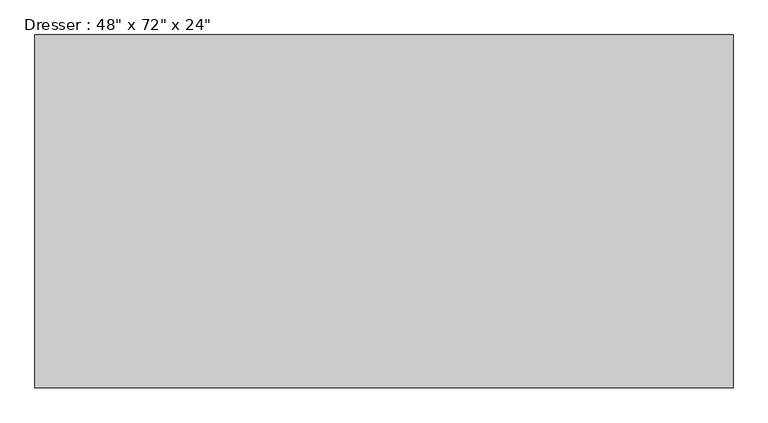
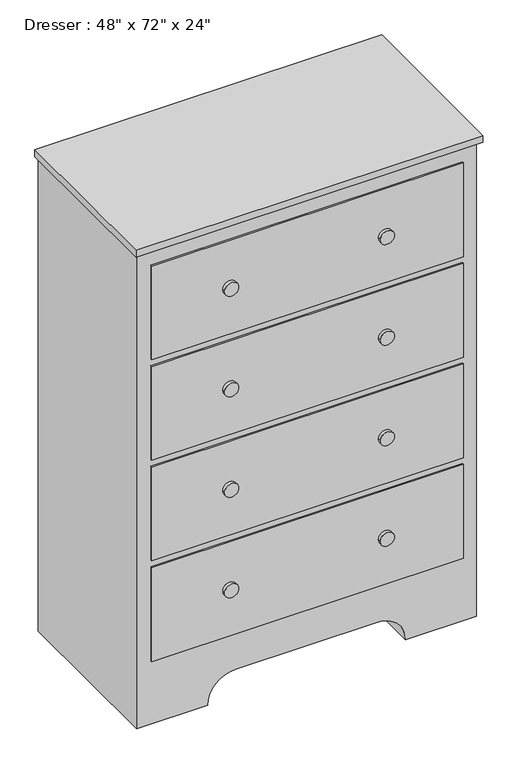
"""IFC4 building model written with IfcOpenShell, lengths in millimetres: furniture geometry."""

from ifc_helpers import new_model, si_unit, point, frame, frame_2d, origin, place, context, project, spatial, polyline, circle_curve, trimmed, segment, composite_curve, outline, extrude, source, transform, mapped, element, save


def furniture_c196debe(model_context):
    return source(origin(), model_context, "Body", "SweptSolid", [
        extrude(outline(composite_curve([segment(polyline([(0.0, 340.4067402), (1803.4, 340.4067402), (1803.4, -878.7932598), (0.0, -878.7932598), (0.0, -624.7932598)]), True, "CONTINUOUS"), segment(trimmed(circle_curve(frame_2d((0.0, -523.1932598)), 101.6), [point((0.0, -624.7932598))], [point((101.6, -523.1932598))], True, "CARTESIAN"), True, "CONTINUOUS"), segment(polyline([(101.6, -523.1932598), (101.6, -15.1932598)]), True, "CONTINUOUS"), segment(trimmed(circle_curve(frame_2d((0.0, -15.1932598)), 101.6), [point((101.6, -15.1932598))], [point((0.0, 86.4067402))], True, "CARTESIAN"), True, "CONTINUOUS"), segment(polyline([(0.0, 86.4067402), (0.0, 340.4067402)]), True, "CONTINUOUS")], self_intersect=False)), frame((0.0, -667.9629541, 0.0), z_axis=(0.0, 1.0, 0.0), x_axis=(0.0, 0.0, 1.0)), (0.0, 0.0, 1.0), 609.6),
        extrude(outline(polyline([(353.1067402, -58.3629541), (353.1067402, -687.0129541), (-891.4932598, -687.0129541), (-891.4932598, -58.3629541), (353.1067402, -58.3629541)])), frame((0.0, 0.0, 1803.4), z_axis=(0.0, 0.0, 1.0), x_axis=(1.0, 0.0, 0.0)), (0.0, 0.0, 1.0), 25.4),
        extrude(outline(polyline([(289.6067402, -674.3129541), (-827.9932598, -674.3129541), (-827.9932598, -667.9629541), (289.6067402, -667.9629541), (289.6067402, -674.3129541)])), frame((0.0, 0.0, 1384.3), z_axis=(0.0, 0.0, 1.0), x_axis=(1.0, 0.0, 0.0)), (0.0, 0.0, 1.0), 355.6),
        extrude(outline(polyline([(289.6067402, -674.3129541), (-827.9932598, -674.3129541), (-827.9932598, -667.9629541), (289.6067402, -667.9629541), (289.6067402, -674.3129541)])), frame((0.0, 0.0, 1003.3), z_axis=(0.0, 0.0, 1.0), x_axis=(1.0, 0.0, 0.0)), (0.0, 0.0, 1.0), 355.6),
        extrude(outline(polyline([(289.6067402, -674.3129541), (-827.9932598, -674.3129541), (-827.9932598, -667.9629541), (289.6067402, -667.9629541), (289.6067402, -674.3129541)])), frame((0.0, 0.0, 622.3), z_axis=(0.0, 0.0, 1.0), x_axis=(1.0, 0.0, 0.0)), (0.0, 0.0, 1.0), 355.6),
        extrude(outline(polyline([(289.6067402, -674.3129541), (-827.9932598, -674.3129541), (-827.9932598, -667.9629541), (289.6067402, -667.9629541), (289.6067402, -674.3129541)])), frame((0.0, 0.0, 241.3), z_axis=(0.0, 0.0, 1.0), x_axis=(1.0, 0.0, 0.0)), (0.0, 0.0, 1.0), 355.6),
        extrude(outline(composite_curve([segment(trimmed(circle_curve(frame_2d((1562.1, 10.2067402)), 25.4), [point((1562.1, -15.1932598))], [point((1562.1, 35.6067402))], False, "CARTESIAN"), True, "CONTINUOUS"), segment(trimmed(circle_curve(frame_2d((1562.1, 10.2067402)), 25.4), [point((1562.1, 35.6067402))], [point((1562.1, -15.1932598))], False, "CARTESIAN"), True, "CONTINUOUS")], self_intersect=False)), frame((0.0, -687.0129541, 0.0), z_axis=(0.0, 1.0, 0.0), x_axis=(0.0, 0.0, 1.0)), (0.0, 0.0, 1.0), 12.7),
        extrude(outline(composite_curve([segment(trimmed(circle_curve(frame_2d((1181.1, 10.2067402)), 25.4), [point((1181.1, -15.1932598))], [point((1181.1, 35.6067402))], False, "CARTESIAN"), True, "CONTINUOUS"), segment(trimmed(circle_curve(frame_2d((1181.1, 10.2067402)), 25.4), [point((1181.1, 35.6067402))], [point((1181.1, -15.1932598))], False, "CARTESIAN"), True, "CONTINUOUS")], self_intersect=False)), frame((0.0, -687.0129541, 0.0), z_axis=(0.0, 1.0, 0.0), x_axis=(0.0, 0.0, 1.0)), (0.0, 0.0, 1.0), 12.7),
        extrude(outline(composite_curve([segment(trimmed(circle_curve(frame_2d((800.1, 10.2067402)), 25.4), [point((800.1, -15.1932598))], [point((800.1, 35.6067402))], False, "CARTESIAN"), True, "CONTINUOUS"), segment(trimmed(circle_curve(frame_2d((800.1, 10.2067402)), 25.4), [point((800.1, 35.6067402))], [point((800.1, -15.1932598))], False, "CARTESIAN"), True, "CONTINUOUS")], self_intersect=False)), frame((0.0, -687.0129541, 0.0), z_axis=(0.0, 1.0, 0.0), x_axis=(0.0, 0.0, 1.0)), (0.0, 0.0, 1.0), 12.7),
        extrude(outline(composite_curve([segment(trimmed(circle_curve(frame_2d((419.1, 10.2067402)), 25.4), [point((419.1, -15.1932598))], [point((419.1, 35.6067402))], False, "CARTESIAN"), True, "CONTINUOUS"), segment(trimmed(circle_curve(frame_2d((419.1, 10.2067402)), 25.4), [point((419.1, 35.6067402))], [point((419.1, -15.1932598))], False, "CARTESIAN"), True, "CONTINUOUS")], self_intersect=False)), frame((0.0, -687.0129541, 0.0), z_axis=(0.0, 1.0, 0.0), x_axis=(0.0, 0.0, 1.0)), (0.0, 0.0, 1.0), 12.7),
        extrude(outline(composite_curve([segment(trimmed(circle_curve(frame_2d((419.1, -548.5932598)), 25.4), [point((419.1, -573.9932598))], [point((419.1, -523.1932598))], False, "CARTESIAN"), True, "CONTINUOUS"), segment(trimmed(circle_curve(frame_2d((419.1, -548.5932598)), 25.4), [point((419.1, -523.1932598))], [point((419.1, -573.9932598))], False, "CARTESIAN"), True, "CONTINUOUS")], self_intersect=False)), frame((0.0, -687.0129541, 0.0), z_axis=(0.0, 1.0, 0.0), x_axis=(0.0, 0.0, 1.0)), (0.0, 0.0, 1.0), 12.7),
        extrude(outline(composite_curve([segment(trimmed(circle_curve(frame_2d((800.1, -548.5932598)), 25.4), [point((800.1, -573.9932598))], [point((800.1, -523.1932598))], False, "CARTESIAN"), True, "CONTINUOUS"), segment(trimmed(circle_curve(frame_2d((800.1, -548.5932598)), 25.4), [point((800.1, -523.1932598))], [point((800.1, -573.9932598))], False, "CARTESIAN"), True, "CONTINUOUS")], self_intersect=False)), frame((0.0, -687.0129541, 0.0), z_axis=(0.0, 1.0, 0.0), x_axis=(0.0, 0.0, 1.0)), (0.0, 0.0, 1.0), 12.7),
        extrude(outline(composite_curve([segment(trimmed(circle_curve(frame_2d((1181.1, -548.5932598)), 25.4), [point((1181.1, -573.9932598))], [point((1181.1, -523.1932598))], False, "CARTESIAN"), True, "CONTINUOUS"), segment(trimmed(circle_curve(frame_2d((1181.1, -548.5932598)), 25.4), [point((1181.1, -523.1932598))], [point((1181.1, -573.9932598))], False, "CARTESIAN"), True, "CONTINUOUS")], self_intersect=False)), frame((0.0, -687.0129541, 0.0), z_axis=(0.0, 1.0, 0.0), x_axis=(0.0, 0.0, 1.0)), (0.0, 0.0, 1.0), 12.7),
        extrude(outline(composite_curve([segment(trimmed(circle_curve(frame_2d((1562.1, -548.5932598)), 25.4), [point((1562.1, -573.9932598))], [point((1562.1, -523.1932598))], False, "CARTESIAN"), True, "CONTINUOUS"), segment(trimmed(circle_curve(frame_2d((1562.1, -548.5932598)), 25.4), [point((1562.1, -523.1932598))], [point((1562.1, -573.9932598))], False, "CARTESIAN"), True, "CONTINUOUS")], self_intersect=False)), frame((0.0, -687.0129541, 0.0), z_axis=(0.0, 1.0, 0.0), x_axis=(0.0, 0.0, 1.0)), (0.0, 0.0, 1.0), 12.7),
    ])


if __name__ == "__main__":
    model = new_model("IFC4")
    model_context = context("Model", 3, world=origin())
    ifc_project = project(units=[si_unit("LENGTHUNIT", "METRE", prefix="MILLI")], contexts=[model_context])
    site = spatial("IfcSite", under=ifc_project)
    building = spatial("IfcBuilding", under=site)
    placement = place(None, origin())
    furniture_shape = furniture_c196debe(model_context)
    element("IfcFurniture", 1, ObjectType="Dresser : 48\" x 72\" x 24\"", at=placement, inside=building, context=model_context, shape_type="MappedRepresentation", body=[
        mapped(furniture_shape, transform((0.0, 0.0, 0.0), x_axis=(1.0, 0.0, 0.0), y_axis=(0.0, 1.0, 0.0), z_axis=(0.0, 0.0, 1.0))),
    ])
    save(model, "model.ifc")

# Revit data of these elements
# Type "Dresser : 48\" x 72\" x 24\""
#   Assembly Code = "E2020200"
#   Depth = 2' - 0"
#   Height = 6' - 0"
#   Width = 4' - 0"
#   Dresser Material = Laminate - Ivory, Glossy
#   Drawer Material = Laminate, Ivory, Matte
#   Knob Material = Cherry
#   Default Elevation = 0
# Element 1 (IfcFurniture, "Dresser : 48\" x 72\" x 24\"")
#   Materials on its faces: "Laminate, Ivory, Matte", "Cherry", "Laminate - Ivory, Glossy"
# Materials
#   "Laminate - Ivory, Glossy": class "Miscellaneous", colour RGB 247 247 239, transparency 0
#   "Laminate, Ivory, Matte": class "Plastic", colour RGB 247 247 239, transparency 0, Description = "Plastic Laminate - Ivory, Matte", Cost = 0
#   "Cherry": class "Wood", colour RGB 233 182 144, transparency 0, Description = "Prunus Serotina", Cost = 0
